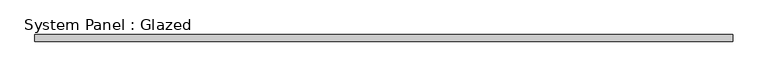
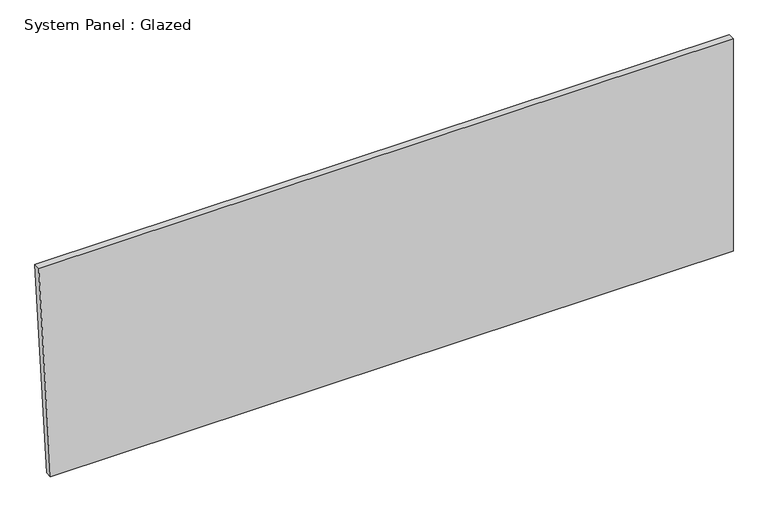
"""IFC4 building model written with IfcOpenShell, lengths in millimetres: plate geometry, System Panel : Glazed."""

from ifc_helpers import new_model, si_unit, frame, origin, place, context, project, spatial, polyline, outline, extrude, source, transform, mapped, element, save


def system_panel_glazed_52faa4d2(model_context):
    return source(origin(), model_context, "Body", "SweptSolid", [
        extrude(outline(polyline([(0.0, -1293.230316), (0.0, 1338.5575225), (866.081558, 1338.5575225), (866.081558, -1338.5575225), (0.0, -1293.230316)])), frame((0.0, -44.45, 0.0), z_axis=(0.0, 1.0, 0.0), x_axis=(0.0, 0.0, 1.0)), (0.0, 0.0, 1.0), 25.4),
    ])


if __name__ == "__main__":
    model = new_model("IFC4")
    model_context = context("Model", 3, world=origin())
    ifc_project = project(units=[si_unit("LENGTHUNIT", "METRE", prefix="MILLI")], contexts=[model_context])
    site = spatial("IfcSite", under=ifc_project)
    building = spatial("IfcBuilding", under=site)
    placement = place(None, origin())
    system_panel_glazed_shape = system_panel_glazed_52faa4d2(model_context)
    element("IfcPlate", 1, ObjectType="System Panel : Glazed", at=placement, inside=building, context=model_context, shape_type="MappedRepresentation", body=[
        mapped(system_panel_glazed_shape, transform((0.0, 0.0, 0.0), x_axis=(1.0, 0.0, 0.0), y_axis=(0.0, 1.0, 0.0), z_axis=(0.0, 0.0, 1.0))),
    ])
    save(model, "model.ifc")

# Revit data of these elements
# Type "System Panel : Glazed"
#   Construction Type Id = "GSP4R"
#   Analytic Construction = "1/8 in Pilkington single glazing"
#   Visual Light Transmittance = 0.9
#   Solar Heat Gain Coefficient = 0.86
#   Heat Transfer Coefficient (U) = 1.18115 BTU/(h·ft²·°F)
#   Define Thermal Properties by = 1
# Element 1 (IfcPlate, "System Panel : Glazed")
#   Materials on its faces: "Glass"
# Materials
#   "Glass": class "Glass", colour RGB 0 128 192, transparency 0.75, Description = "Soda Lime Glass", Cost = 0
